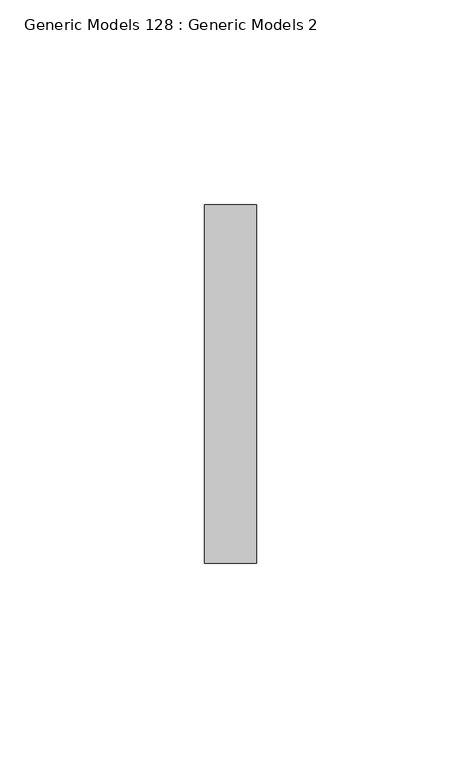
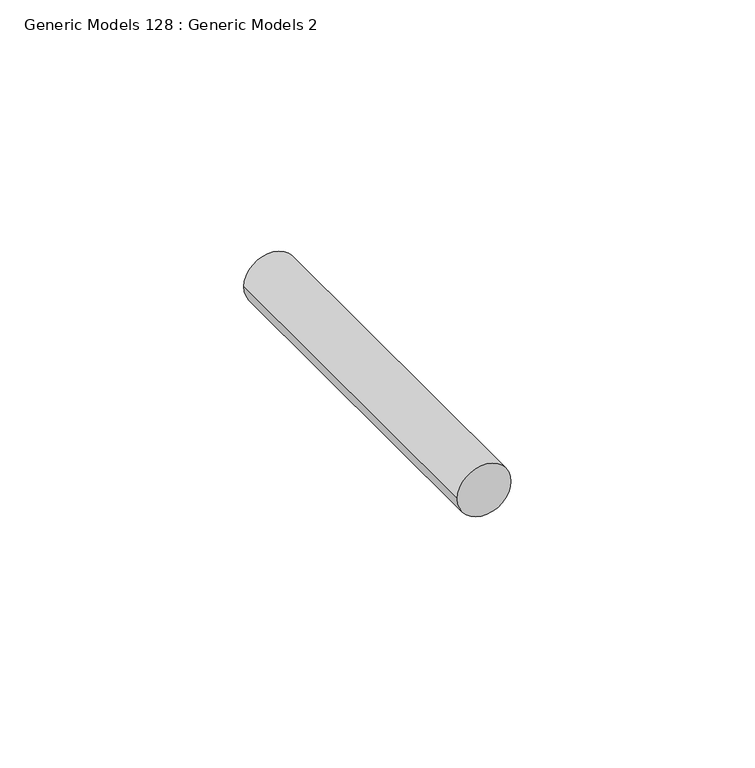
"""IFC4 building model written with IfcOpenShell, lengths in millimetres: proxy geometry, Generic Models 128 : Generic Models 2."""

import ifcopenshell
import ifcopenshell.guid

model = None  # the IFC model being written
_history = None  # IfcOwnerHistory: only IFC2X3 demands one
_inside = {}  # id of a spatial element -> (the spatial element, [elements in it])
_under = {}  # id of a project, library or spatial element -> (it, [spatial elements below it])
_declared = {}  # id of a project -> (the project, [libraries it declares])
_typed = {}  # id of a type object -> (the type object, [elements of that type])
_made_of = {}  # id of a material, layer set ... -> (it, [elements and type objects made of it])


def new_model(schema):
    """Start an empty IFC model of exactly this schema.

    Asked for "IFC4X3", IfcOpenShell would pick the latest addendum, in which some entities
    have other attributes; the version numbers below select the first issue.
    IFC2X3 requires an IfcOwnerHistory on every rooted entity: one is made here for all.
    """
    global model, _history
    if schema == "IFC4X3":
        model = ifcopenshell.file(schema_version=(4, 3, 0, 0))
    else:
        model = ifcopenshell.file(schema=schema)
    _inside.clear()
    _under.clear()
    _declared.clear()
    _typed.clear()
    _made_of.clear()
    _history = None
    if model.schema == "IFC2X3":
        org = make("IfcOrganization", Name="unknown")
        user = make(
            "IfcPersonAndOrganization",
            ThePerson=make("IfcPerson", FamilyName="unknown"),
            TheOrganization=org,
        )
        app = make(
            "IfcApplication",
            ApplicationDeveloper=org,
            Version="unknown",
            ApplicationFullName="unknown",
            ApplicationIdentifier="unknown",
        )
        _history = make(
            "IfcOwnerHistory",
            OwningUser=user,
            OwningApplication=app,
            ChangeAction="ADDED",
            CreationDate=0,
        )
    return model


def make(cls, **values):
    """One entity of the class cls with the attributes given. An attribute that is None is left unset."""
    return model.create_entity(
        cls, **{name: value for name, value in values.items() if value is not None}
    )


def rooted(cls, **values):
    """An entity with a GlobalId (a new one), such as an element, a storey or a relation."""
    return make(cls, GlobalId=ifcopenshell.guid.new(), OwnerHistory=_history, **values)


def si_unit(unit_type, name, prefix=None):
    """IfcSIUnit, for example si_unit("LENGTHUNIT", "METRE", prefix="MILLI")."""
    return make("IfcSIUnit", UnitType=unit_type, Prefix=prefix, Name=name)


def assignment(units):
    """IfcUnitAssignment: the units of a project."""
    return None if units is None else make("IfcUnitAssignment", Units=units)


def point(xyz):
    """IfcCartesianPoint."""
    return None if xyz is None else make("IfcCartesianPoint", Coordinates=xyz)


def direction(xyz):
    """IfcDirection."""
    return None if xyz is None else make("IfcDirection", DirectionRatios=xyz)


def frame(location, z_axis=None, x_axis=None):
    """IfcAxis2Placement3D, a coordinate frame: its origin and axes. An axis left out is left unset."""
    return make(
        "IfcAxis2Placement3D",
        Location=point(location),
        Axis=direction(z_axis),
        RefDirection=direction(x_axis),
    )


def frame_2d(location, x_axis=None):
    """IfcAxis2Placement2D, a coordinate frame in the plane: its origin and x axis."""
    return make(
        "IfcAxis2Placement2D", Location=point(location), RefDirection=direction(x_axis)
    )


def origin():
    """The frame at (0, 0, 0) with its axes left unset."""
    return frame((0.0, 0.0, 0.0))


def place(relative_to, where):
    """IfcLocalPlacement: puts the frame where relative to a parent placement (None: the world)."""
    return make(
        "IfcLocalPlacement", PlacementRelTo=relative_to, RelativePlacement=where
    )


def context(
    kind, dimensions, precision=None, world=None, true_north=None, identifier=None
):
    """IfcGeometricRepresentationContext, for example the 3D "Model" context."""
    return make(
        "IfcGeometricRepresentationContext",
        ContextIdentifier=identifier,
        ContextType=kind,
        CoordinateSpaceDimension=dimensions,
        Precision=precision,
        WorldCoordinateSystem=world,
        TrueNorth=true_north,
    )


def project(units=None, contexts=None):
    """IfcProject with its units and contexts."""
    return rooted(
        "IfcProject",
        Name="project",
        RepresentationContexts=contexts,
        UnitsInContext=assignment(units),
    )


def spatial(cls, under=None, at=None, **own):
    """A site, building, storey or space (cls), placed at a placement, below another one or the project."""
    s = rooted(cls, ObjectPlacement=at, **own)
    if under is not None:
        _under.setdefault(under.id(), (under, []))[1].append(s)
    return s


def circle_curve(where, radius):
    """IfcCircle in the frame where."""
    return make("IfcCircle", Position=where, Radius=radius)


def trimmed(basis, trim1, trim2, sense, master):
    """IfcTrimmedCurve: the piece of a basis curve between two trims."""
    return make(
        "IfcTrimmedCurve",
        BasisCurve=basis,
        Trim1=trim1,
        Trim2=trim2,
        SenseAgreement=sense,
        MasterRepresentation=master,
    )


def segment(curve, same_sense, transition):
    """IfcCompositeCurveSegment."""
    return make(
        "IfcCompositeCurveSegment",
        Transition=transition,
        SameSense=same_sense,
        ParentCurve=curve,
    )


def composite_curve(segments, self_intersect=None):
    """IfcCompositeCurve: segments joined end to end."""
    return make("IfcCompositeCurve", Segments=segments, SelfIntersect=self_intersect)


def outline(outer, holes=None, kind="AREA"):
    """IfcArbitraryClosedProfileDef: a profile drawn as a closed curve; with holes, ...WithVoids."""
    if holes is None:
        return make("IfcArbitraryClosedProfileDef", ProfileType=kind, OuterCurve=outer)
    return make(
        "IfcArbitraryProfileDefWithVoids",
        ProfileType=kind,
        OuterCurve=outer,
        InnerCurves=holes,
    )


def extrude(swept, where, along, depth):
    """IfcExtrudedAreaSolid: the profile swept, set in the frame where, extruded along a direction by depth."""
    return make(
        "IfcExtrudedAreaSolid",
        SweptArea=swept,
        Position=where,
        ExtrudedDirection=direction(along),
        Depth=depth,
    )


def shape(context_of_items, identifier, shape_type, items):
    """IfcShapeRepresentation: the items that make up one representation, for example the "Body"."""
    return make(
        "IfcShapeRepresentation",
        ContextOfItems=context_of_items,
        RepresentationIdentifier=identifier,
        RepresentationType=shape_type,
        Items=items,
    )


def source(mapping_origin, context_of_items, identifier, shape_type, items):
    """IfcRepresentationMap: a shape defined once, which mapped items show again and again."""
    return make(
        "IfcRepresentationMap",
        MappingOrigin=mapping_origin,
        MappedRepresentation=shape(context_of_items, identifier, shape_type, items),
    )


def transform(
    local_origin,
    x_axis=None,
    y_axis=None,
    z_axis=None,
    scale=None,
    scale2=None,
    scale3=None,
    uniform=True,
):
    """IfcCartesianTransformationOperator3D, or its non-uniform kind. x_axis, y_axis, z_axis: its Axis1, 2, 3."""
    if uniform:
        return make(
            "IfcCartesianTransformationOperator3D",
            Axis1=direction(x_axis),
            Axis2=direction(y_axis),
            LocalOrigin=point(local_origin),
            Scale=scale,
            Axis3=direction(z_axis),
        )
    return make(
        "IfcCartesianTransformationOperator3DnonUniform",
        Axis1=direction(x_axis),
        Axis2=direction(y_axis),
        LocalOrigin=point(local_origin),
        Scale=scale,
        Axis3=direction(z_axis),
        Scale2=scale2,
        Scale3=scale3,
    )


def mapped(mapping_source, mapping_target):
    """IfcMappedItem: shows the shape of a source again, moved by a transform."""
    return make(
        "IfcMappedItem", MappingSource=mapping_source, MappingTarget=mapping_target
    )


def made_of(thing, what):
    """Note that an element or type object is made of a material, layer set ...; save() writes the relation."""
    if what is not None:
        _made_of.setdefault(what.id(), (what, []))[1].append(thing)
    return thing


def element(
    cls,
    number,
    at=None,
    inside=None,
    cuts=None,
    type_object=None,
    material=None,
    context=None,
    identifier="Body",
    shape_type=None,
    held_by="IfcProductDefinitionShape",
    body=None,
    shapes=None,
    **own,
):
    """One element of the class cls, such as IfcWall. Its Tag is "e" and its number.

    at: its placement. inside: the storey or other place that contains it. cuts: it is an
    opening in that element (IfcRelVoidsElement). A single representation is given by context,
    identifier, shape_type and body (its items); several are given by shapes. held_by: the class
    of the entity that holds the representations. save() writes the other relations.
    """
    e = rooted(cls, Tag="e%d" % number, ObjectPlacement=at, **own)
    if body is not None:
        shapes = [shape(context, identifier, shape_type, body)]
    if shapes is not None:
        e.Representation = make(held_by, Representations=shapes)
    if inside is not None:
        _inside.setdefault(inside.id(), (inside, []))[1].append(e)
    if cuts is not None:
        rooted(
            "IfcRelVoidsElement", RelatingBuildingElement=cuts, RelatedOpeningElement=e
        )
    if type_object is not None:
        _typed.setdefault(type_object.id(), (type_object, []))[1].append(e)
    return made_of(e, material)


def aggregate(whole, parts):
    """IfcRelAggregates: a whole, such as a stair, and the parts it consists of."""
    return rooted("IfcRelAggregates", RelatingObject=whole, RelatedObjects=parts)


def save(model, path):
    """Write the relations noted so far, then the file.

    IfcRelAggregates (storeys below a building ...), IfcRelContainedInSpatialStructure (elements
    in a storey), IfcRelDefinesByType, IfcRelAssociatesMaterial and IfcRelDeclares: one each for
    every whole, place, type object, material and project.
    """
    for whole, parts in _under.values():
        aggregate(whole, parts)
    for where, things in _inside.values():
        rooted(
            "IfcRelContainedInSpatialStructure",
            RelatedElements=things,
            RelatingStructure=where,
        )
    for kind, things in _typed.values():
        rooted("IfcRelDefinesByType", RelatedObjects=things, RelatingType=kind)
    for what, things in _made_of.values():
        rooted("IfcRelAssociatesMaterial", RelatedObjects=things, RelatingMaterial=what)
    for by, libraries in _declared.values():
        rooted("IfcRelDeclares", RelatingContext=by, RelatedDefinitions=libraries)
    model.write(path)


def generic_models_128_generic_models_2_581f5a26(model_context):
    return source(origin(), model_context, "Body", "SweptSolid", [
        extrude(outline(composite_curve([segment(trimmed(circle_curve(frame_2d((38374.9548538, 7576.9346014)), 6.35), [point((38374.9548538, 7583.2846014))], [point((38374.9548538, 7570.5846014))], False, "CARTESIAN"), True, "CONTINUOUS"), segment(trimmed(circle_curve(frame_2d((38374.9548538, 7576.9346014)), 6.35), [point((38374.9548538, 7570.5846014))], [point((38374.9548538, 7583.2846014))], False, "CARTESIAN"), True, "CONTINUOUS")], self_intersect=False)), frame((0.0, 1848.3666731, 0.0), z_axis=(0.0, 1.0, 0.0), x_axis=(0.0, 0.0, 1.0)), (0.0, 0.0, 1.0), 87.551022),
    ])


if __name__ == "__main__":
    model = new_model("IFC4")
    model_context = context("Model", 3, world=origin())
    ifc_project = project(units=[si_unit("LENGTHUNIT", "METRE", prefix="MILLI")], contexts=[model_context])
    site = spatial("IfcSite", under=ifc_project)
    building = spatial("IfcBuilding", under=site)
    placement = place(None, origin())
    generic_models_128_generic_models_2_shape = generic_models_128_generic_models_2_581f5a26(model_context)
    element("IfcBuildingElementProxy", 1, Name="Generic Models 128 : Generic Models 2", ObjectType="Generic Models 128 : Generic Models 2", at=placement, inside=building, context=model_context, shape_type="MappedRepresentation", body=[
        mapped(generic_models_128_generic_models_2_shape, transform((0.0, 0.0, 0.0), x_axis=(1.0, 0.0, 0.0), y_axis=(0.0, 1.0, 0.0), z_axis=(0.0, 0.0, 1.0))),
    ])
    save(model, "model.ifc")

# Revit data of these elements
# Element 1 (IfcBuildingElementProxy, "Generic Models 128 : Generic Models 2")
#   Materials on its faces: "S.S. LAG BOLT - SEE STRUCT. DWGS"
# Materials
#   "S.S. LAG BOLT - SEE STRUCT. DWGS": class "Generic", colour RGB 120 120 120, transparency 0, Cost = 0
